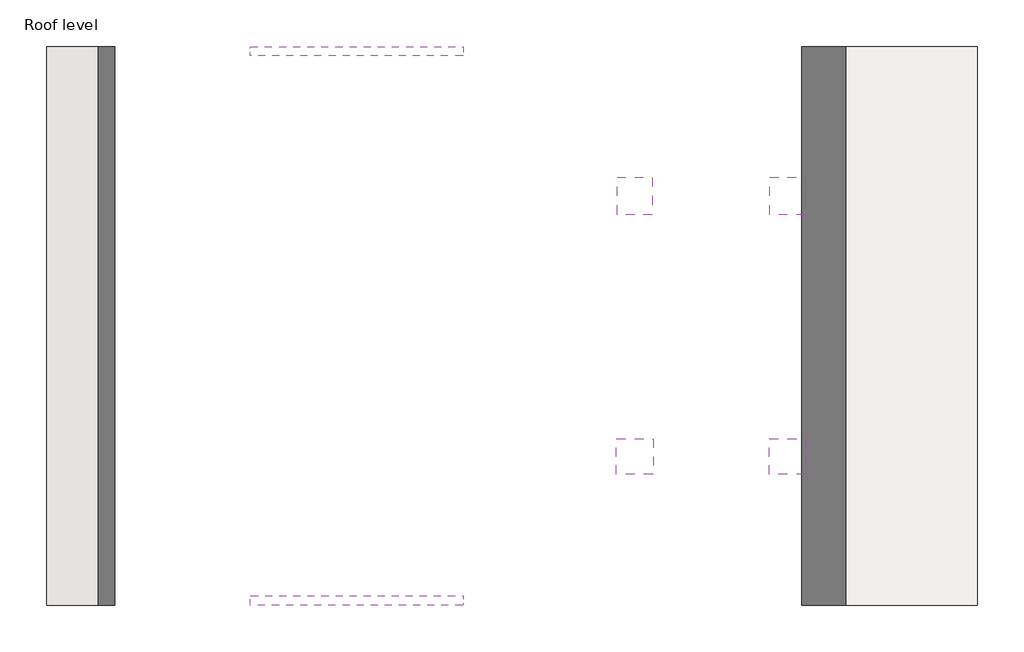
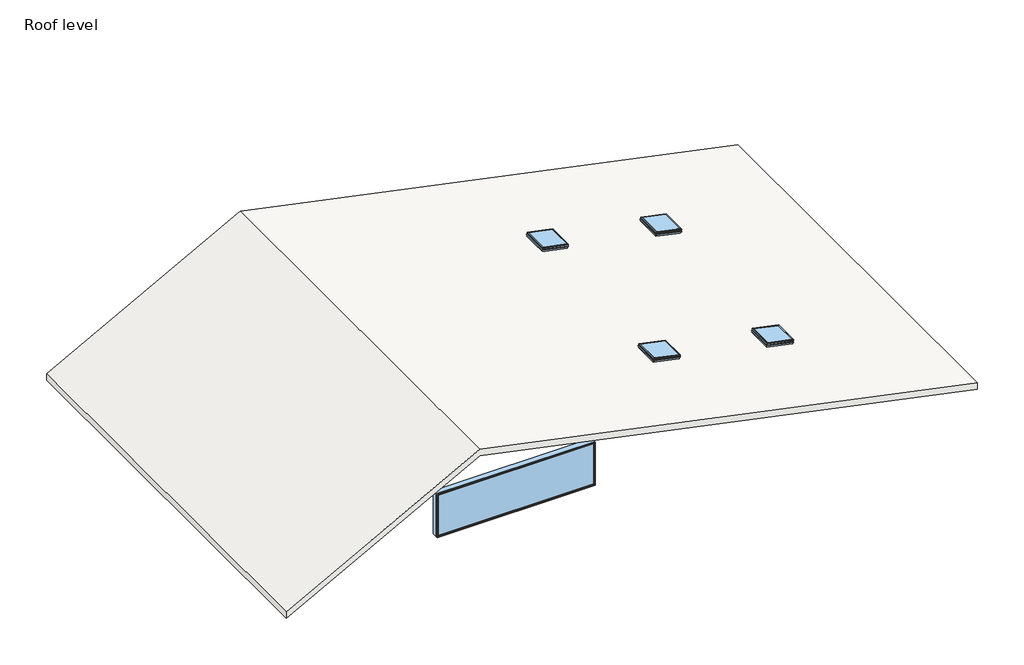
# One storey: 6 windows, 1 roof.
"""IFC4 building model written with IfcOpenShell, lengths in millimetres."""

import ifcopenshell
import ifcopenshell.guid

model = None  # the IFC model being written
_history = None  # IfcOwnerHistory: only IFC2X3 demands one
_inside = {}  # id of a spatial element -> (the spatial element, [elements in it])
_under = {}  # id of a project, library or spatial element -> (it, [spatial elements below it])
_declared = {}  # id of a project -> (the project, [libraries it declares])
_typed = {}  # id of a type object -> (the type object, [elements of that type])
_made_of = {}  # id of a material, layer set ... -> (it, [elements and type objects made of it])


def new_model(schema):
    """Start an empty IFC model of exactly this schema.

    Asked for "IFC4X3", IfcOpenShell would pick the latest addendum, in which some entities
    have other attributes; the version numbers below select the first issue.
    IFC2X3 requires an IfcOwnerHistory on every rooted entity: one is made here for all.
    """
    global model, _history
    if schema == "IFC4X3":
        model = ifcopenshell.file(schema_version=(4, 3, 0, 0))
    else:
        model = ifcopenshell.file(schema=schema)
    _inside.clear()
    _under.clear()
    _declared.clear()
    _typed.clear()
    _made_of.clear()
    _history = None
    if model.schema == "IFC2X3":
        org = make("IfcOrganization", Name="unknown")
        user = make(
            "IfcPersonAndOrganization",
            ThePerson=make("IfcPerson", FamilyName="unknown"),
            TheOrganization=org,
        )
        app = make(
            "IfcApplication",
            ApplicationDeveloper=org,
            Version="unknown",
            ApplicationFullName="unknown",
            ApplicationIdentifier="unknown",
        )
        _history = make(
            "IfcOwnerHistory",
            OwningUser=user,
            OwningApplication=app,
            ChangeAction="ADDED",
            CreationDate=0,
        )
    return model


def make(cls, **values):
    """One entity of the class cls with the attributes given. An attribute that is None is left unset."""
    return model.create_entity(
        cls, **{name: value for name, value in values.items() if value is not None}
    )


def rooted(cls, **values):
    """An entity with a GlobalId (a new one), such as an element, a storey or a relation."""
    return make(cls, GlobalId=ifcopenshell.guid.new(), OwnerHistory=_history, **values)


def si_unit(unit_type, name, prefix=None):
    """IfcSIUnit, for example si_unit("LENGTHUNIT", "METRE", prefix="MILLI")."""
    return make("IfcSIUnit", UnitType=unit_type, Prefix=prefix, Name=name)


def assignment(units):
    """IfcUnitAssignment: the units of a project."""
    return None if units is None else make("IfcUnitAssignment", Units=units)


def point(xyz):
    """IfcCartesianPoint."""
    return None if xyz is None else make("IfcCartesianPoint", Coordinates=xyz)


def direction(xyz):
    """IfcDirection."""
    return None if xyz is None else make("IfcDirection", DirectionRatios=xyz)


def frame(location, z_axis=None, x_axis=None):
    """IfcAxis2Placement3D, a coordinate frame: its origin and axes. An axis left out is left unset."""
    return make(
        "IfcAxis2Placement3D",
        Location=point(location),
        Axis=direction(z_axis),
        RefDirection=direction(x_axis),
    )


def origin():
    """The frame at (0, 0, 0) with its axes left unset."""
    return frame((0.0, 0.0, 0.0))


def place(relative_to, where):
    """IfcLocalPlacement: puts the frame where relative to a parent placement (None: the world)."""
    return make(
        "IfcLocalPlacement", PlacementRelTo=relative_to, RelativePlacement=where
    )


def context(
    kind, dimensions, precision=None, world=None, true_north=None, identifier=None
):
    """IfcGeometricRepresentationContext, for example the 3D "Model" context."""
    return make(
        "IfcGeometricRepresentationContext",
        ContextIdentifier=identifier,
        ContextType=kind,
        CoordinateSpaceDimension=dimensions,
        Precision=precision,
        WorldCoordinateSystem=world,
        TrueNorth=true_north,
    )


def project(units=None, contexts=None):
    """IfcProject with its units and contexts."""
    return rooted(
        "IfcProject",
        Name="project",
        RepresentationContexts=contexts,
        UnitsInContext=assignment(units),
    )


def spatial(cls, under=None, at=None, **own):
    """A site, building, storey or space (cls), placed at a placement, below another one or the project."""
    s = rooted(cls, ObjectPlacement=at, **own)
    if under is not None:
        _under.setdefault(under.id(), (under, []))[1].append(s)
    return s


def polyline(points):
    """IfcPolyline through the points."""
    return make("IfcPolyline", Points=[point(p) for p in points])


def outline(outer, holes=None, kind="AREA"):
    """IfcArbitraryClosedProfileDef: a profile drawn as a closed curve; with holes, ...WithVoids."""
    if holes is None:
        return make("IfcArbitraryClosedProfileDef", ProfileType=kind, OuterCurve=outer)
    return make(
        "IfcArbitraryProfileDefWithVoids",
        ProfileType=kind,
        OuterCurve=outer,
        InnerCurves=holes,
    )


def extrude(swept, where, along, depth):
    """IfcExtrudedAreaSolid: the profile swept, set in the frame where, extruded along a direction by depth."""
    return make(
        "IfcExtrudedAreaSolid",
        SweptArea=swept,
        Position=where,
        ExtrudedDirection=direction(along),
        Depth=depth,
    )


def faces_of(points, faces, orient=None, outer=None):
    """IfcFace entities. A face is a list of loops; a loop is a list of indices into points, from 0.

    orient and outer hold one flag for each loop. By default every Orientation is true, the
    first loop of a face is its IfcFaceOuterBound and the others are IfcFaceBound.
    """
    made = []
    for i, loops in enumerate(faces):
        bounds = []
        for j, loop in enumerate(loops):
            is_outer = j == 0 if outer is None else outer[i][j]
            bounds.append(
                make(
                    "IfcFaceOuterBound" if is_outer else "IfcFaceBound",
                    Bound=make("IfcPolyLoop", Polygon=[points[k] for k in loop]),
                    Orientation=True if orient is None else orient[i][j],
                )
            )
        made.append(make("IfcFace", Bounds=bounds))
    return made


def faceted_brep(points, faces, orient=None, outer=None, voids=None):
    """IfcFacetedBrep: a solid bounded by flat faces; with voids (closed shells), ...WithVoids."""
    shared = [point(p) for p in points]
    hull = make("IfcClosedShell", CfsFaces=faces_of(shared, faces, orient, outer))
    if voids is None:
        return make("IfcFacetedBrep", Outer=hull)
    return make(
        "IfcFacetedBrepWithVoids",
        Outer=hull,
        Voids=[
            make(cls, CfsFaces=faces_of(shared, fs, o, b)) for cls, fs, o, b in voids
        ],
    )


def shape(context_of_items, identifier, shape_type, items):
    """IfcShapeRepresentation: the items that make up one representation, for example the "Body"."""
    return make(
        "IfcShapeRepresentation",
        ContextOfItems=context_of_items,
        RepresentationIdentifier=identifier,
        RepresentationType=shape_type,
        Items=items,
    )


def source(mapping_origin, context_of_items, identifier, shape_type, items):
    """IfcRepresentationMap: a shape defined once, which mapped items show again and again."""
    return make(
        "IfcRepresentationMap",
        MappingOrigin=mapping_origin,
        MappedRepresentation=shape(context_of_items, identifier, shape_type, items),
    )


def transform(
    local_origin,
    x_axis=None,
    y_axis=None,
    z_axis=None,
    scale=None,
    scale2=None,
    scale3=None,
    uniform=True,
):
    """IfcCartesianTransformationOperator3D, or its non-uniform kind. x_axis, y_axis, z_axis: its Axis1, 2, 3."""
    if uniform:
        return make(
            "IfcCartesianTransformationOperator3D",
            Axis1=direction(x_axis),
            Axis2=direction(y_axis),
            LocalOrigin=point(local_origin),
            Scale=scale,
            Axis3=direction(z_axis),
        )
    return make(
        "IfcCartesianTransformationOperator3DnonUniform",
        Axis1=direction(x_axis),
        Axis2=direction(y_axis),
        LocalOrigin=point(local_origin),
        Scale=scale,
        Axis3=direction(z_axis),
        Scale2=scale2,
        Scale3=scale3,
    )


def mapped(mapping_source, mapping_target):
    """IfcMappedItem: shows the shape of a source again, moved by a transform."""
    return make(
        "IfcMappedItem", MappingSource=mapping_source, MappingTarget=mapping_target
    )


def made_of(thing, what):
    """Note that an element or type object is made of a material, layer set ...; save() writes the relation."""
    if what is not None:
        _made_of.setdefault(what.id(), (what, []))[1].append(thing)
    return thing


def element(
    cls,
    number,
    at=None,
    inside=None,
    cuts=None,
    type_object=None,
    material=None,
    context=None,
    identifier="Body",
    shape_type=None,
    held_by="IfcProductDefinitionShape",
    body=None,
    shapes=None,
    **own,
):
    """One element of the class cls, such as IfcWall. Its Tag is "e" and its number.

    at: its placement. inside: the storey or other place that contains it. cuts: it is an
    opening in that element (IfcRelVoidsElement). A single representation is given by context,
    identifier, shape_type and body (its items); several are given by shapes. held_by: the class
    of the entity that holds the representations. save() writes the other relations.
    """
    e = rooted(cls, Tag="e%d" % number, ObjectPlacement=at, **own)
    if body is not None:
        shapes = [shape(context, identifier, shape_type, body)]
    if shapes is not None:
        e.Representation = make(held_by, Representations=shapes)
    if inside is not None:
        _inside.setdefault(inside.id(), (inside, []))[1].append(e)
    if cuts is not None:
        rooted(
            "IfcRelVoidsElement", RelatingBuildingElement=cuts, RelatedOpeningElement=e
        )
    if type_object is not None:
        _typed.setdefault(type_object.id(), (type_object, []))[1].append(e)
    return made_of(e, material)


def aggregate(whole, parts):
    """IfcRelAggregates: a whole, such as a stair, and the parts it consists of."""
    return rooted("IfcRelAggregates", RelatingObject=whole, RelatedObjects=parts)


def save(model, path):
    """Write the relations noted so far, then the file.

    IfcRelAggregates (storeys below a building ...), IfcRelContainedInSpatialStructure (elements
    in a storey), IfcRelDefinesByType, IfcRelAssociatesMaterial and IfcRelDeclares: one each for
    every whole, place, type object, material and project.
    """
    for whole, parts in _under.values():
        aggregate(whole, parts)
    for where, things in _inside.values():
        rooted(
            "IfcRelContainedInSpatialStructure",
            RelatedElements=things,
            RelatingStructure=where,
        )
    for kind, things in _typed.values():
        rooted("IfcRelDefinesByType", RelatedObjects=things, RelatingType=kind)
    for what, things in _made_of.values():
        rooted("IfcRelAssociatesMaterial", RelatedObjects=things, RelatingMaterial=what)
    for by, libraries in _declared.values():
        rooted("IfcRelDeclares", RelatingContext=by, RelatedDefinitions=libraries)
    model.write(path)


def m_fixed_2800x4977mm_04857461(model_context):
    return source(origin(), model_context, "Body", "SweptSolid", [
        extrude(outline(polyline([(-3420.85, 130.4), (3420.85, 130.4), (3420.85, 118.4), (-3420.85, 118.4), (-3420.85, 130.4)])), frame((0.0, 0.0, 978.0), z_axis=(0.0, 0.0, 1.0), x_axis=(1.0, 0.0, 0.0)), (0.0, 0.0, 1.0), 1874.0),
        extrude(outline(polyline([(2896.0, -3464.85), (934.0, -3464.85), (934.0, 3464.85), (2896.0, 3464.85), (2896.0, -3464.85)]), holes=[polyline([(2852.0, -3420.85), (2852.0, 3420.85), (978.0, 3420.85), (978.0, -3420.85), (2852.0, -3420.85)])]), frame((0.0, 102.4, 0.0), z_axis=(0.0, 1.0, 0.0), x_axis=(0.0, 0.0, 1.0)), (0.0, 0.0, 1.0), 44.0),
        extrude(outline(polyline([(2915.0, -3483.85), (915.0, -3483.85), (915.0, 3483.85), (2915.0, 3483.85), (2915.0, -3483.85)]), holes=[polyline([(2896.0, -3464.85), (2896.0, 3464.85), (934.0, 3464.85), (934.0, -3464.85), (2896.0, -3464.85)])]), frame((0.0, 102.4, 0.0), z_axis=(0.0, 1.0, 0.0), x_axis=(0.0, 0.0, 1.0)), (0.0, 0.0, 1.0), 63.0),
        extrude(outline(polyline([(2915.0, -3483.85), (915.0, -3483.85), (915.0, 3483.85), (2915.0, 3483.85), (2915.0, -3483.85)]), holes=[polyline([(2883.0, -3451.85), (2883.0, 3451.85), (947.0, 3451.85), (947.0, -3451.85), (2883.0, -3451.85)])]), frame((0.0, -139.4, 0.0), z_axis=(0.0, 1.0, 0.0), x_axis=(0.0, 0.0, 1.0)), (0.0, 0.0, 1.0), 241.8),
    ])


def m_fixed_2800x4977mm_bf86b0e8(model_context):
    return source(origin(), model_context, "Body", "SweptSolid", [
        extrude(outline(polyline([(-3420.85, -130.4), (-3420.85, -118.4), (3420.85, -118.4), (3420.85, -130.4), (-3420.85, -130.4)])), frame((0.0, 0.0, 978.0), z_axis=(0.0, 0.0, 1.0), x_axis=(1.0, 0.0, 0.0)), (0.0, 0.0, 1.0), 1874.0),
        extrude(outline(polyline([(2896.0, -3464.85), (934.0, -3464.85), (934.0, 3464.85), (2896.0, 3464.85), (2896.0, -3464.85)]), holes=[polyline([(2852.0, -3420.85), (2852.0, 3420.85), (978.0, 3420.85), (978.0, -3420.85), (2852.0, -3420.85)])]), frame((0.0, -146.4, 0.0), z_axis=(0.0, 1.0, 0.0), x_axis=(0.0, 0.0, 1.0)), (0.0, 0.0, 1.0), 44.0),
        extrude(outline(polyline([(2915.0, -3483.85), (915.0, -3483.85), (915.0, 3483.85), (2915.0, 3483.85), (2915.0, -3483.85)]), holes=[polyline([(2896.0, -3464.85), (2896.0, 3464.85), (934.0, 3464.85), (934.0, -3464.85), (2896.0, -3464.85)])]), frame((0.0, -165.4, 0.0), z_axis=(0.0, 1.0, 0.0), x_axis=(0.0, 0.0, 1.0)), (0.0, 0.0, 1.0), 63.0),
        extrude(outline(polyline([(2915.0, -3483.85), (915.0, -3483.85), (915.0, 3483.85), (2915.0, 3483.85), (2915.0, -3483.85)]), holes=[polyline([(2883.0, -3451.85), (2883.0, 3451.85), (947.0, 3451.85), (947.0, -3451.85), (2883.0, -3451.85)])]), frame((0.0, -102.4, 0.0), z_axis=(0.0, 1.0, 0.0), x_axis=(0.0, 0.0, 1.0)), (0.0, 0.0, 1.0), 241.8),
    ])


def window_c0717641(model_context):
    return source(origin(), model_context, "Body", "SolidModel", [
        faceted_brep([(254.440073, 370.1040988, 4114.8), (279.840073, 395.5040988, 4114.8), (279.840073, -772.8959012, 4114.8), (254.440073, -747.4959012, 4114.8), (254.440073, 370.1040988, 4140.2), (254.440073, -747.4959012, 4140.2), (292.540073, 408.2040988, 4140.2), (292.540073, -785.5959012, 4140.2), (292.540073, 408.2040988, 4114.8), (292.540073, -785.5959012, 4114.8), (292.540073, 408.2040988, 4064.0), (292.540073, -785.5959012, 4064.0), (307.1089145, 422.7729403, 4043.1935381), (307.1089145, -800.1647427, 4043.1935381), (301.907299, 417.5713248, 4039.5513277), (301.907299, -794.9631272, 4039.5513277), (286.190073, 401.8540988, 4061.9978527), (286.190073, -779.2459012, 4061.9978527), (286.190073, 401.8540988, 4114.8), (286.190073, -779.2459012, 4114.8), (-837.759927, -772.8959012, 4114.8), (-812.359927, -747.4959012, 4114.8), (-812.359927, -747.4959012, 4140.2), (-850.459927, -785.5959012, 4140.2), (-850.459927, -785.5959012, 4114.8), (-850.459927, -785.5959012, 4064.0), (-865.0287685, -800.1647427, 4043.1935381), (-859.827153, -794.9631272, 4039.5513277), (-844.109927, -779.2459012, 4061.9978527), (-844.109927, -779.2459012, 4114.8), (-837.759927, 395.5040988, 4114.8), (-812.359927, 370.1040988, 4114.8), (-812.359927, 370.1040988, 4140.2), (-850.459927, 408.2040988, 4140.2), (-850.459927, 408.2040988, 4114.8), (-850.459927, 408.2040988, 4064.0), (-865.0287685, 422.7729403, 4043.1935381), (-859.827153, 417.5713248, 4039.5513277), (-844.109927, 401.8540988, 4061.9978527), (-844.109927, 401.8540988, 4114.8)], [[[0, 1, 2, 3]], [[4, 0, 3, 5]], [[6, 4, 5, 7]], [[8, 6, 7, 9]], [[10, 8, 9, 11]], [[12, 10, 11, 13]], [[14, 12, 13, 15]], [[16, 14, 15, 17]], [[18, 16, 17, 19]], [[1, 18, 19, 2]], [[3, 2, 20, 21]], [[5, 3, 21, 22]], [[7, 5, 22, 23]], [[9, 7, 23, 24]], [[11, 9, 24, 25]], [[13, 11, 25, 26]], [[15, 13, 26, 27]], [[17, 15, 27, 28]], [[19, 17, 28, 29]], [[2, 19, 29, 20]], [[21, 20, 30, 31]], [[22, 21, 31, 32]], [[23, 22, 32, 33]], [[24, 23, 33, 34]], [[25, 24, 34, 35]], [[26, 25, 35, 36]], [[27, 26, 36, 37]], [[28, 27, 37, 38]], [[29, 28, 38, 39]], [[20, 29, 39, 30]], [[31, 30, 1, 0]], [[32, 31, 0, 4]], [[33, 32, 4, 6]], [[34, 33, 6, 8]], [[35, 34, 8, 10]], [[36, 35, 10, 12]], [[37, 36, 12, 14]], [[38, 37, 14, 16]], [[39, 38, 16, 18]], [[30, 39, 18, 1]]]),
        faceted_brep([(279.840073, -772.8959012, 4114.8), (279.840073, -772.8959012, 3962.4), (279.840073, 395.5040988, 3962.4), (279.840073, 395.5040988, 4114.8), (254.440073, -747.4959012, 4114.8), (254.440073, 370.1040988, 4114.8), (254.440073, -747.4959012, 4089.4), (254.440073, 370.1040988, 4089.4), (235.390073, -728.4459012, 4089.4), (235.390073, 351.0540988, 4089.4), (235.390073, -728.4459012, 3962.4), (235.390073, 351.0540988, 3962.4), (-837.759927, 395.5040988, 3962.4), (-837.759927, 395.5040988, 4114.8), (-812.359927, 370.1040988, 4114.8), (-812.359927, 370.1040988, 4089.4), (-793.309927, 351.0540988, 4089.4), (-793.309927, 351.0540988, 3962.4), (-837.759927, -772.8959012, 3962.4), (-837.759927, -772.8959012, 4114.8), (-812.359927, -747.4959012, 4114.8), (-812.359927, -747.4959012, 4089.4), (-793.309927, -728.4459012, 4089.4), (-793.309927, -728.4459012, 3962.4)], [[[0, 1, 2, 3]], [[4, 0, 3, 5]], [[6, 4, 5, 7]], [[8, 6, 7, 9]], [[10, 8, 9, 11]], [[1, 10, 11, 2]], [[3, 2, 12, 13]], [[5, 3, 13, 14]], [[7, 5, 14, 15]], [[9, 7, 15, 16]], [[11, 9, 16, 17]], [[2, 11, 17, 12]], [[13, 12, 18, 19]], [[14, 13, 19, 20]], [[15, 14, 20, 21]], [[16, 15, 21, 22]], [[17, 16, 22, 23]], [[12, 17, 23, 18]], [[19, 18, 1, 0]], [[20, 19, 0, 4]], [[21, 20, 4, 6]], [[22, 21, 6, 8]], [[23, 22, 8, 10]], [[18, 23, 10, 1]]]),
        extrude(outline(polyline([(254.440073, -747.4959012), (-812.359927, -747.4959012), (-812.359927, 370.1040988), (254.440073, 370.1040988), (254.440073, -747.4959012)])), frame((0.0, 0.0, 4133.85), z_axis=(0.0, 0.0, 1.0), x_axis=(1.0, 0.0, 0.0)), (0.0, 0.0, 1.0), 6.35),
    ])


model = new_model("IFC4")

# Units and contexts
model_context = context("Model", 3, world=origin())
ifc_project = project(units=[si_unit("LENGTHUNIT", "METRE", prefix="MILLI")], contexts=[model_context])

# Site, building, storey
site = spatial("IfcSite", under=ifc_project)
building = spatial("IfcBuilding", under=site)
storey = spatial("IfcBuildingStorey", under=building, Name="Roof level", Elevation=9144.0)

# Roof
placement = place(None, origin())
element("IfcRoof", 1, ObjectType="Generic Roof - 304.8mm", at=placement, inside=storey, context=model_context, shape_type="Brep", body=[
    faceted_brep([(31657.0035739, 12383.3990339, 9448.8), (31657.0035739, 12383.3990339, 9144.0), (9711.4035739, 12383.3990339, 13716.0), (1177.0035739, 12383.3990339, 9144.0), (1177.0035739, 12383.3990339, 9448.8), (9711.4035739, 12383.3990339, 14020.8), (1177.0035739, -5904.6009661, 9144.0), (1177.0035739, -5904.6009661, 9448.8), (9711.4035739, -5904.6009661, 13716.0), (31657.0035739, -5904.6009661, 9144.0), (31657.0035739, -5904.6009661, 9448.8), (9711.4035739, -5904.6009661, 14020.8), (25945.0342483, -1554.3509661, 10638.7936095), (24888.2248852, -1554.3509661, 10858.9622268), (24888.2248852, -525.6509661, 10858.9622268), (25945.0342483, -525.6509661, 10638.7936095), (25920.1681456, 8033.1490339, 10643.9740476), (25920.1681456, 6953.6490339, 10643.9740476), (24913.0909878, 6953.6490339, 10853.7817888), (24913.0909878, 8033.1490339, 10853.7817888), (20920.1681456, 8033.1490339, 11685.6407142), (20920.1681456, 6953.6490339, 11685.6407142), (19913.0909878, 6953.6490339, 11895.4484554), (19913.0909878, 8033.1490339, 11895.4484554), (20945.0342483, -1554.3509661, 11680.4602762), (19888.2248852, -1554.3509661, 11900.6288935), (19888.2248852, -525.6509661, 11900.6288935), (20945.0342483, -525.6509661, 11680.4602762), (24827.3663161, -1554.3509661, 10566.8410954), (25884.1756792, -1554.3509661, 10346.6724781), (25884.1756792, -525.6509661, 10346.6724781), (24827.3663161, -525.6509661, 10566.8410954), (25859.3095765, 6953.6490339, 10351.8529161), (25859.3095765, 8033.1490339, 10351.8529161), (24852.2324188, 8033.1490339, 10561.6606573), (24852.2324188, 6953.6490339, 10561.6606573), (20859.3095765, 6953.6490339, 11393.5195828), (20859.3095765, 8033.1490339, 11393.5195828), (19852.2324188, 8033.1490339, 11603.327324), (19852.2324188, 6953.6490339, 11603.327324), (19827.3663161, -1554.3509661, 11608.507762), (20884.1756792, -1554.3509661, 11388.3391447), (20884.1756792, -525.6509661, 11388.3391447), (19827.3663161, -525.6509661, 11608.507762)], [[[0, 1, 2, 3, 4, 5]], [[4, 3, 6, 7]], [[7, 6, 8, 9, 10, 11]], [[1, 0, 10, 9]], [[4, 7, 11, 5]], [[6, 3, 2, 8]], [[10, 0, 5, 11], [12, 13, 14, 15], [16, 17, 18, 19], [20, 21, 22, 23], [24, 25, 26, 27]], [[1, 9, 8, 2], [28, 29, 30, 31], [32, 33, 34, 35], [36, 37, 38, 39], [40, 41, 42, 43]], [[12, 29, 28, 13]], [[13, 28, 31, 14]], [[14, 31, 30, 15]], [[29, 12, 15, 30]], [[16, 33, 32, 17]], [[17, 32, 35, 18]], [[18, 35, 34, 19]], [[33, 16, 19, 34]], [[20, 37, 36, 21]], [[21, 36, 39, 22]], [[22, 39, 38, 23]], [[37, 20, 23, 38]], [[24, 41, 40, 25]], [[25, 40, 43, 26]], [[26, 43, 42, 27]], [[41, 24, 27, 42]]]),
])

# Windows
m_fixed_2800x4977mm_shape = m_fixed_2800x4977mm_04857461(model_context)
element("IfcWindow", 2, ObjectType="M_Fixed : 2800X4977mm", at=placement, inside=storey, context=model_context, shape_type="MappedRepresentation", body=[
    mapped(m_fixed_2800x4977mm_shape, transform((11329.4035739, 12217.9990339, 9644.0), x_axis=(1.0, 0.0, 0.0), y_axis=(0.0, 1.0, 0.0), z_axis=(0.0, 0.0, 1.0))),
])
m_fixed_2800x4977mm_2_shape = m_fixed_2800x4977mm_bf86b0e8(model_context)
element("IfcWindow", 3, ObjectType="M_Fixed : 2800X4977mm", at=placement, inside=storey, context=model_context, shape_type="MappedRepresentation", body=[
    mapped(m_fixed_2800x4977mm_2_shape, transform((11329.4035739, -5739.2009661, 9644.0), x_axis=(1.0, 0.0, 0.0), y_axis=(0.0, 1.0, 0.0), z_axis=(0.0, 0.0, 1.0))),
])
window_shape = window_c0717641(model_context)
element("IfcWindow", 4, ObjectType="Skylight : 44\" x 46\"", at=placement, inside=storey, context=model_context, shape_type="MappedRepresentation", body=[
    mapped(window_shape, transform((24794.5175104, -1318.9608931, 6837.5526717), x_axis=(0.0, -1.0000000000000004, 0.0), y_axis=(0.9789804197376053, 0.0, -0.2039542541120017), z_axis=(0.2039542541120016, 0.0, 0.9789804197376049))),
])
element("IfcWindow", 5, ObjectType="Skylight : 44\" x 46\"", at=placement, inside=storey, context=model_context, shape_type="MappedRepresentation", body=[
    mapped(window_shape, transform((24882.8842242, 7682.0949351, 6819.1429396), x_axis=(0.9789804197376049, 0.0, -0.20395425411200158), y_axis=(0.0, 1.0, 0.0), z_axis=(0.20395425411200158, 0.0, 0.978980419737605))),
])
element("IfcWindow", 6, ObjectType="Skylight : 44\" x 46\"", at=placement, inside=storey, context=model_context, shape_type="MappedRepresentation", body=[
    mapped(window_shape, transform((19794.5175104, -1318.9608931, 7879.2193384), x_axis=(0.0, -1.0000000000000004, 0.0), y_axis=(0.9789804197376053, 0.0, -0.2039542541120017), z_axis=(0.2039542541120016, 0.0, 0.9789804197376049))),
])
element("IfcWindow", 7, ObjectType="Skylight : 44\" x 46\"", at=placement, inside=storey, context=model_context, shape_type="MappedRepresentation", body=[
    mapped(window_shape, transform((19882.8842242, 7682.0949351, 7860.8096063), x_axis=(0.9789804197376049, 0.0, -0.20395425411200158), y_axis=(0.0, 1.0, 0.0), z_axis=(0.20395425411200158, 0.0, 0.978980419737605))),
])

save(model, "model.ifc")

# Revit data of these elements
# Type "Generic Roof - 304.8mm"
#   Layers, outside or top first: 304.8 mm no material (function 1)
# Type "M_Fixed : 2800X4977mm"
#   Type Mark = "29"
#   Height = 2000 mm
#   Default Sill Height = 915 mm
#   Width = 6967.7 mm
#   Window Inset = 19 mm
#   Frame Exterior Material = Sash
#   Frame Interior Material = Sash
#   Glass Pane Material = Glass
#   Sash = Sash
#   Wall Closure = (empty or 0)
# Type "Skylight : 44\" x 46\""
#   Type Mark = "50"
#   Construction Type Id = "GSP4R"
#   Assembly Code = "B3020110"
#   Analytic Construction = "1/8 in Pilkington single glazing"
#   Visual Light Transmittance = 0.9
#   Solar Heat Gain Coefficient = 0.78
#   Heat Transfer Coefficient (U) = 3.6886 W/(m²·K)
#   Height = 1168.4 mm
#   Width = 1117.6 mm
#   Glass Pane = Glass
#   Frame Material = Metal - Bronze, Light Brush
#   Type Comments = ""
# Element 1 (IfcRoof, "Generic Roof - 304.8mm")
#   built-in parameter 1001705 = 31 (stored number, unit not read)
#   built-in parameter 1001710 = 33615
#   Phase Created = New Construction
#   Materials on its faces: "Default Roof"
# Element 2 (IfcWindow, "M_Fixed : 2800X4977mm")
#   Mark = "91"
#   Phase Created = New Construction
#   Materials on its faces: "Sash", "Glass"
# Element 3 (IfcWindow, "M_Fixed : 2800X4977mm")
#   Mark = "93"
#   Phase Created = New Construction
#   Materials on its faces: "Sash", "Glass"
# Element 4 (IfcWindow, "Skylight : 44\" x 46\"")
#   Mark = "1"
#   Phase Created = New Construction
#   Materials on its faces: "Metal - Bronze, Light Brush", "Glass"
# Element 5 (IfcWindow, "Skylight : 44\" x 46\"")
#   Mark = "3"
#   Phase Created = New Construction
#   Materials on its faces: "Metal - Bronze, Light Brush", "Glass"
# Element 6 (IfcWindow, "Skylight : 44\" x 46\"")
#   Mark = "4"
#   Phase Created = New Construction
#   Materials on its faces: "Metal - Bronze, Light Brush", "Glass"
# Element 7 (IfcWindow, "Skylight : 44\" x 46\"")
#   Mark = "5"
#   Phase Created = New Construction
#   Materials on its faces: "Metal - Bronze, Light Brush", "Glass"
# Materials
#   "Sash": class "Wood", colour RGB 136 99 55, transparency 0
#   "Glass": class "Glass", colour RGB 0 128 192, transparency 0.9, Description = "Soda Lime Glass", Cost = 0
#   "Metal - Bronze, Light Brush": class "Metal", colour RGB 113 80 70, transparency 0
#   "Default Roof": class "Miscellaneous", colour RGB 0 127 0, transparency 0, Cost = 0
